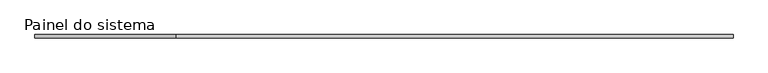
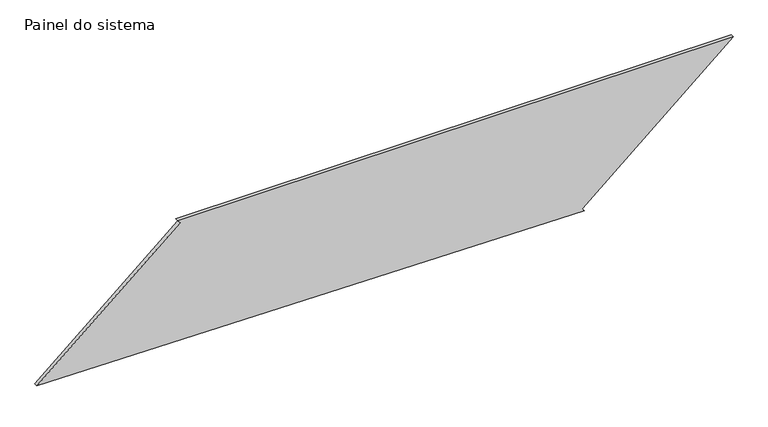
"""IFC4 building model written with IfcOpenShell, lengths in millimetres: plate geometry, Painel do sistema : Envidraçado."""

from ifc_helpers import new_model, si_unit, frame, origin, place, context, project, spatial, polyline, outline, extrude, source, transform, mapped, element, save


def painel_do_sistema_8f47ad2b(model_context):
    return source(origin(), model_context, "Body", "SweptSolid", [
        extrude(outline(polyline([(0.0, 1408.1965805), (19.0100862, 1391.9603056), (929.9876704, 2458.5696398), (929.9876704, -1464.172723), (910.9775842, -1447.9364481), (47.8085175, -2458.5696398), (0.0, 1408.1965805)])), frame((0.0, 24.5, 0.0), z_axis=(0.0, 1.0, 0.0), x_axis=(0.0, 0.0, 1.0)), (0.0, 0.0, 1.0), 25.0),
    ])


if __name__ == "__main__":
    model = new_model("IFC4")
    model_context = context("Model", 3, world=origin())
    ifc_project = project(units=[si_unit("LENGTHUNIT", "METRE", prefix="MILLI")], contexts=[model_context])
    site = spatial("IfcSite", under=ifc_project)
    building = spatial("IfcBuilding", under=site)
    placement = place(None, origin())
    painel_do_sistema_shape = painel_do_sistema_8f47ad2b(model_context)
    element("IfcPlate", 1, ObjectType="Painel do sistema : Envidraçado", at=placement, inside=building, context=model_context, shape_type="MappedRepresentation", body=[
        mapped(painel_do_sistema_shape, transform((0.0, 0.0, 0.0), x_axis=(1.0, 0.0, 0.0), y_axis=(0.0, 1.0, 0.0), z_axis=(0.0, 0.0, 1.0))),
    ])
    save(model, "model.ifc")

# Revit data of these elements
# Type "Painel do sistema : Envidraçado"
#   Construction Type Id = "GSP4R"
#   Analytic Construction = "Vidraça única Pilkington 1/8 pol"
#   Visual Light Transmittance = 0.9
#   Solar Heat Gain Coefficient = 0.86
#   Heat Transfer Coefficient (U) = 6.7069 W/(m²·K)
# Element 1 (IfcPlate, "Painel do sistema : Envidraçado")
#   Materials on its faces: "Vidro"
# Materials
#   "Vidro": class "Vidro", colour RGB 0 128 192, transparency 0.9, Description = "Vidro de sílica", Cost = 0
